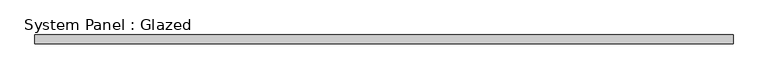
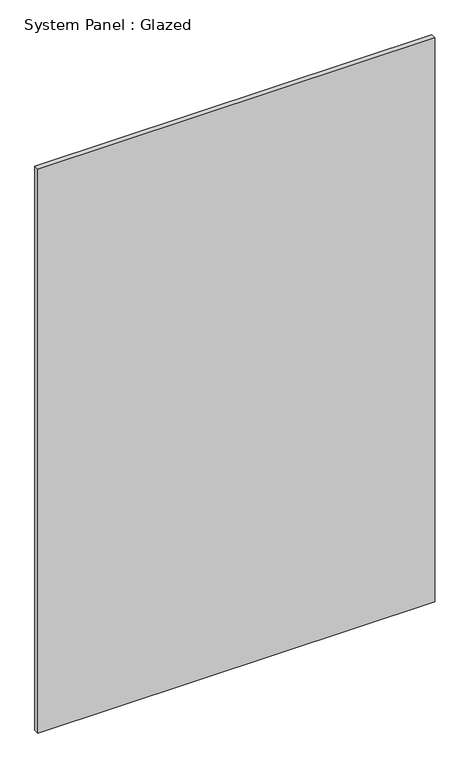
"""IFC4 building model written with IfcOpenShell, lengths in millimetres: plate geometry, System Panel : Glazed."""

from ifc_helpers import new_model, si_unit, origin, origin_with_axes, place, context, project, spatial, polyline, outline, extrude, source, transform, mapped, element, save


def system_panel_glazed_e38ee6be(model_context):
    return source(origin(), model_context, "Body", "SweptSolid", [
        extrude(outline(polyline([(974.1833333, 24.5), (-974.1833333, 24.5), (-974.1833333, 49.5), (974.1833333, 49.5), (974.1833333, 24.5)])), origin_with_axes(), (0.0, 0.0, 1.0), 2925.0),
    ])


if __name__ == "__main__":
    model = new_model("IFC4")
    model_context = context("Model", 3, world=origin())
    ifc_project = project(units=[si_unit("LENGTHUNIT", "METRE", prefix="MILLI")], contexts=[model_context])
    site = spatial("IfcSite", under=ifc_project)
    building = spatial("IfcBuilding", under=site)
    placement = place(None, origin())
    system_panel_glazed_shape = system_panel_glazed_e38ee6be(model_context)
    element("IfcPlate", 1, ObjectType="System Panel : Glazed", at=placement, inside=building, context=model_context, shape_type="MappedRepresentation", body=[
        mapped(system_panel_glazed_shape, transform((0.0, 0.0, 0.0), x_axis=(1.0, 0.0, 0.0), y_axis=(0.0, 1.0, 0.0), z_axis=(0.0, 0.0, 1.0))),
    ])
    save(model, "model.ifc")

# Revit data of these elements
# Element 1 (IfcPlate, "System Panel : Glazed")
#   Materials on its faces: "Glass"
# Materials
#   "Glass": class "Glass", colour RGB 0 128 192, transparency 0.9
